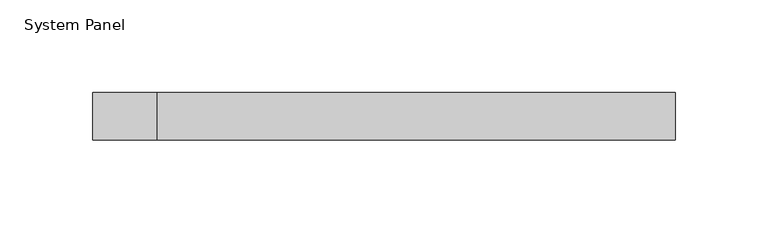
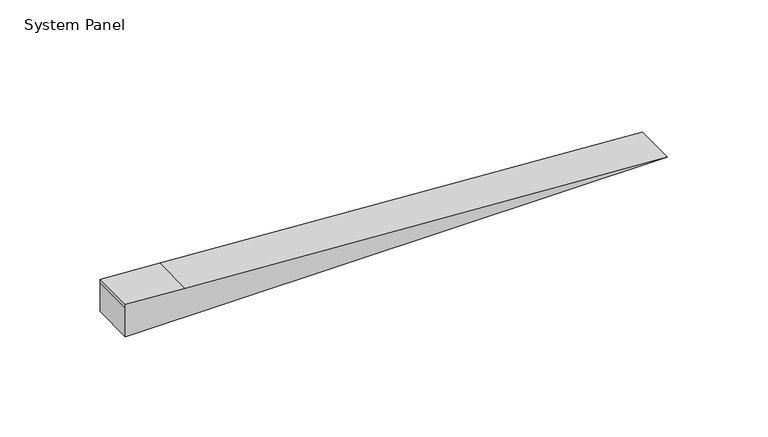
"""IFC4 building model written with IfcOpenShell, lengths in millimetres: plate geometry, System Panel : TEMPERED INSULATED GLAZING (CARDINAL GLASS LoĒ²-240."""

from ifc_helpers import new_model, si_unit, frame, origin, place, context, project, spatial, polyline, outline, extrude, source, transform, mapped, element, save


def system_panel_0570641b(model_context):
    return source(origin(), model_context, "Body", "SweptSolid", [
        extrude(outline(polyline([(0.0, -156.5619671), (0.0, 156.5619671), (17.4056663, -121.9286939), (19.5702459, -156.5619671), (17.4056663, -156.5619671), (0.0, -156.5619671)])), frame((0.0, 6.35, 0.0), z_axis=(0.0, 1.0, 0.0), x_axis=(0.0, 0.0, 1.0)), (0.0, 0.0, 1.0), 25.4),
    ])


if __name__ == "__main__":
    model = new_model("IFC4")
    model_context = context("Model", 3, world=origin())
    ifc_project = project(units=[si_unit("LENGTHUNIT", "METRE", prefix="MILLI")], contexts=[model_context])
    site = spatial("IfcSite", under=ifc_project)
    building = spatial("IfcBuilding", under=site)
    placement = place(None, origin())
    system_panel_shape = system_panel_0570641b(model_context)
    element("IfcPlate", 1, ObjectType="System Panel : TEMPERED INSULATED GLAZING (CARDINAL GLASS LoĒ²-240", at=placement, inside=building, context=model_context, shape_type="MappedRepresentation", body=[
        mapped(system_panel_shape, transform((0.0, 0.0, 0.0), x_axis=(1.0, 0.0, 0.0), y_axis=(0.0, 1.0, 0.0), z_axis=(0.0, 0.0, 1.0))),
    ])
    save(model, "model.ifc")

# Revit data of these elements
# Type "System Panel : TEMPERED INSULATED GLAZING (CARDINAL GLASS LoĒ²-240"
#   Construction Type Id = "opn-s72"
#   Analytic Construction = "Double glazing - 1/4 in thick - low-E/clear (e = 0.1) glass"
#   Visual Light Transmittance = 0.72
#   Solar Heat Gain Coefficient = 0.6
#   Heat Transfer Coefficient (U) = 1.9873 W/(m²·K)
#   Transparency_Hack = 70
# Element 1 (IfcPlate, "System Panel : TEMPERED INSULATED GLAZING (CARDINAL GLASS LoĒ²-240")
#   Materials on its faces: "TEMPERED INSULATED GLAZING (CARDINAL GLASS LoĒ²-240\nOR EQUIVALENT)"
# Materials
#   "TEMPERED INSULATED GLAZING (CARDINAL GLASS LoĒ²-240\nOR EQUIVALENT)": class "Glass", colour RGB 196 205 210, transparency 0.85, Description = "Soda Lime Glass", Cost = 0
